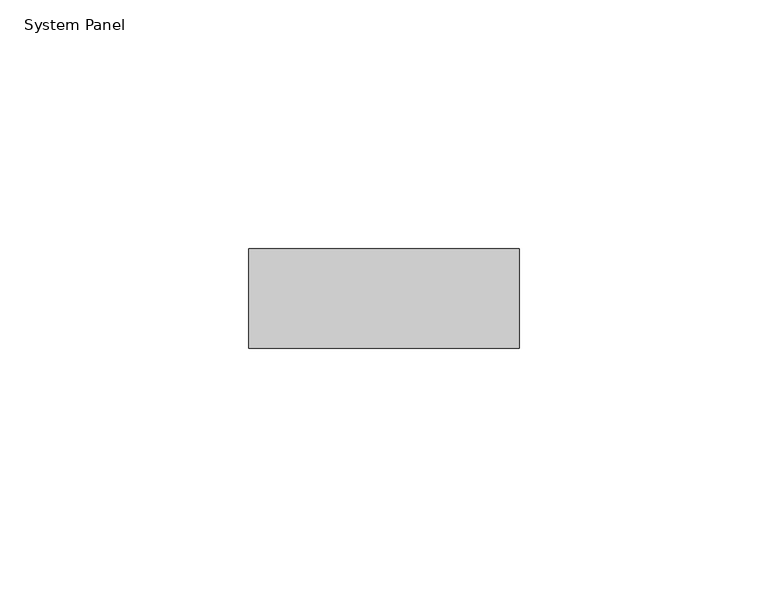
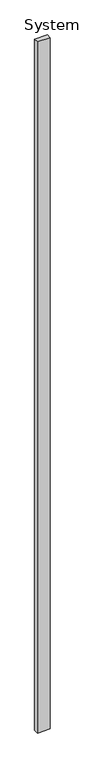
"""IFC4 building model written with IfcOpenShell, lengths in millimetres: plate geometry, System Panel : WWm-Glass-20mm-10mmOffset."""

from ifc_helpers import new_model, si_unit, origin, origin_with_axes, place, context, project, spatial, polyline, outline, extrude, source, transform, mapped, element, save


def system_panel_7736fef0(model_context):
    return source(origin(), model_context, "Body", "SweptSolid", [
        extrude(outline(polyline([(27.1729644, 0.0), (-27.1729644, 0.0), (-27.1729644, 20.0), (27.1729644, 20.0), (27.1729644, 0.0)])), origin_with_axes(), (0.0, 0.0, 1.0), 3150.0),
    ])


if __name__ == "__main__":
    model = new_model("IFC4")
    model_context = context("Model", 3, world=origin())
    ifc_project = project(units=[si_unit("LENGTHUNIT", "METRE", prefix="MILLI")], contexts=[model_context])
    site = spatial("IfcSite", under=ifc_project)
    building = spatial("IfcBuilding", under=site)
    placement = place(None, origin())
    system_panel_shape = system_panel_7736fef0(model_context)
    element("IfcPlate", 1, ObjectType="System Panel : WWm-Glass-20mm-10mmOffset", at=placement, inside=building, context=model_context, shape_type="MappedRepresentation", body=[
        mapped(system_panel_shape, transform((0.0, 0.0, 0.0), x_axis=(1.0, 0.0, 0.0), y_axis=(0.0, 1.0, 0.0), z_axis=(0.0, 0.0, 1.0))),
    ])
    save(model, "model.ifc")

# Revit data of these elements
# Type "System Panel : WWm-Glass-20mm-10mmOffset"
#   Finish = ""
# Element 1 (IfcPlate, "System Panel : WWm-Glass-20mm-10mmOffset")
#   Materials on its faces: "WW-EC-GL-Storefront"
# Materials
#   "WW-EC-GL-Storefront": class "Glass", colour RGB 236 240 239, transparency 0.85, Description = "Storefront Glass", Cost = 0
